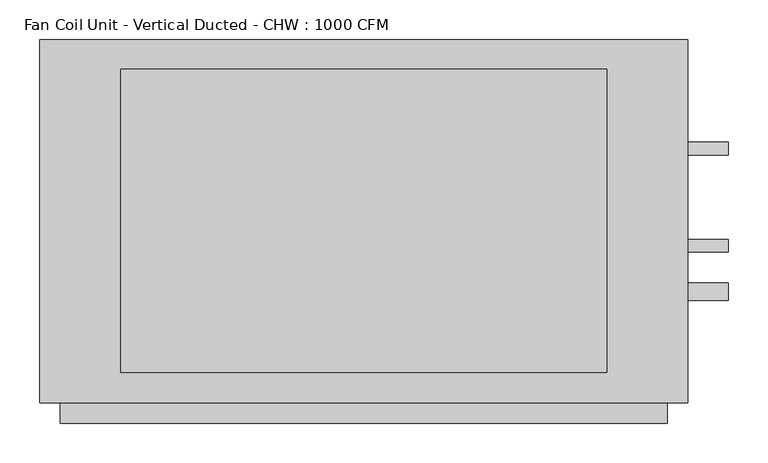
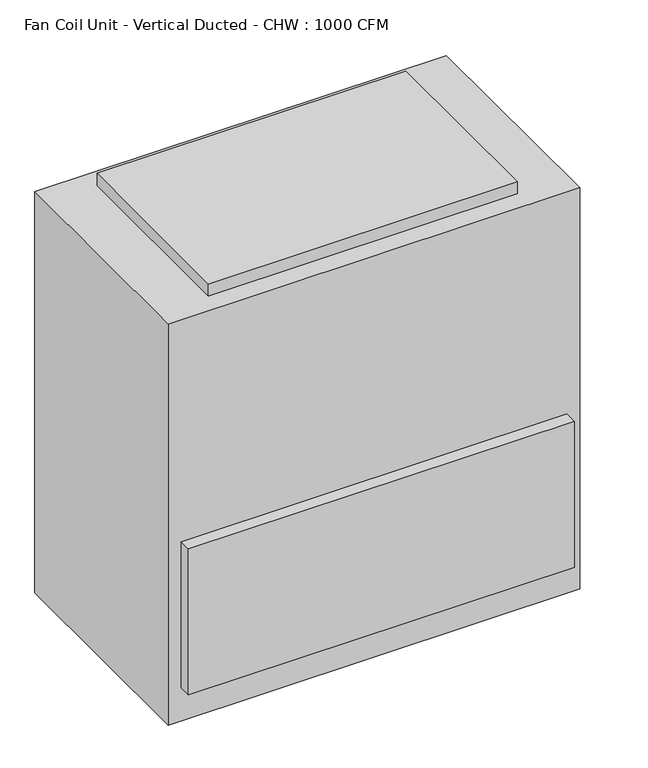
"""IFC4 building model written with IfcOpenShell, lengths in millimetres: proxy geometry, Fan Coil Unit - Vertical Ducted - CHW : 1000 CFM."""

from ifc_helpers import new_model, si_unit, frame, origin, place, context, project, spatial, circle_curve, source, transform, mapped, element, save
from ifc_brep_helpers import plane_surface, cylinder_surface, advanced_brep


def fan_coil_unit_vertical_ducted_chw_1000_cfm_3afe99c5(model_context):
    return source(origin(), model_context, "Body", "AdvancedBrep", [
        advanced_brep(
        [(711.2, 419.1, 863.6), (101.6, 419.1, 863.6), (101.6, 38.1, 863.6), (711.2, 38.1, 863.6), (711.2, 419.1, 838.2), (101.6, 419.1, 838.2), (101.6, 38.1, 838.2), (711.2, 38.1, 838.2), (812.8, 455.901774, 838.2), (0.0, 455.901774, 838.2), (0.0, 0.0, 838.2), (812.8, 0.0, 838.2), (812.8, 455.901774, 0.0), (812.8, 0.0, 0.0), (0.0, 0.0, 0.0), (0.0, 455.901774, 0.0), (25.4, 0.0, 374.65), (787.4, 0.0, 374.65), (787.4, 0.0, 69.85), (25.4, 0.0, 69.85), (812.8, 327.314274, 673.1), (812.8, 311.439274, 673.1), (812.8, 205.076774, 593.725), (812.8, 189.201774, 593.725), (812.8, 150.8125, 431.8), (812.8, 128.5875, 431.8), (787.4, -25.4, 374.65), (25.4, -25.4, 374.65), (25.4, -25.4, 69.85), (787.4, -25.4, 69.85), (863.6, 311.439274, 673.1), (863.6, 327.314274, 673.1), (863.6, 189.201774, 593.725), (863.6, 205.076774, 593.725), (863.6, 128.5875, 431.8), (863.6, 150.8125, 431.8)],
        [
            (0, 1),
            (1, 2),
            (2, 3),
            (3, 0),
            (0, 4),
            (4, 5),
            (5, 1),
            (5, 6),
            (6, 2),
            (6, 7),
            (7, 3),
            (7, 4),
            (8, 9),
            (9, 10),
            (10, 11),
            (11, 8),
            (12, 13),
            (13, 14),
            (14, 15),
            (15, 12),
            (8, 12),
            (15, 9),
            (14, 10),
            (13, 11),
            (16, 17),
            (17, 18),
            (18, 19),
            (19, 16),
            (20, 21, circle_curve(frame((812.8, 319.376774, 673.1), z_axis=(-1.0, 0.0, 0.0), x_axis=(0.0, 1.0, 0.0)), 7.9375)),
            (21, 20, circle_curve(frame((812.8, 319.376774, 673.1), z_axis=(-1.0, 0.0, 0.0), x_axis=(0.0, 1.0, 0.0)), 7.9375)),
            (22, 23, circle_curve(frame((812.8, 197.139274, 593.725), z_axis=(-1.0, 0.0, 0.0), x_axis=(0.0, 1.0, 0.0)), 7.9375)),
            (23, 22, circle_curve(frame((812.8, 197.139274, 593.725), z_axis=(-1.0, 0.0, 0.0), x_axis=(0.0, 1.0, 0.0)), 7.9375)),
            (24, 25, circle_curve(frame((812.8, 139.7, 431.8), z_axis=(-1.0, 0.0, 0.0), x_axis=(0.0, 1.0, 0.0)), 11.1125)),
            (25, 24, circle_curve(frame((812.8, 139.7, 431.8), z_axis=(-1.0, 0.0, 0.0), x_axis=(0.0, 1.0, 0.0)), 11.1125)),
            (26, 27),
            (27, 28),
            (28, 29),
            (29, 26),
            (26, 17),
            (16, 27),
            (19, 28),
            (18, 29),
            (30, 31, circle_curve(frame((863.6, 319.376774, 673.1), z_axis=(1.0, 0.0, 0.0), x_axis=(0.0, 1.0, 0.0)), 7.9375)),
            (31, 30, circle_curve(frame((863.6, 319.376774, 673.1), z_axis=(1.0, 0.0, 0.0), x_axis=(0.0, 1.0, 0.0)), 7.9375)),
            (30, 21),
            (20, 31),
            (32, 33, circle_curve(frame((863.6, 197.139274, 593.725), z_axis=(1.0, 0.0, 0.0), x_axis=(0.0, 1.0, 0.0)), 7.9375)),
            (33, 32, circle_curve(frame((863.6, 197.139274, 593.725), z_axis=(1.0, 0.0, 0.0), x_axis=(0.0, 1.0, 0.0)), 7.9375)),
            (32, 23),
            (22, 33),
            (34, 35, circle_curve(frame((863.6, 139.7, 431.8), z_axis=(1.0, 0.0, 0.0), x_axis=(0.0, 1.0, 0.0)), 11.1125)),
            (35, 34, circle_curve(frame((863.6, 139.7, 431.8), z_axis=(1.0, 0.0, 0.0), x_axis=(0.0, 1.0, 0.0)), 11.1125)),
            (34, 25),
            (24, 35),
        ],
        [
            plane_surface(frame((101.6, 419.1, 863.6), z_axis=(0.0, 0.0, 1.0), x_axis=(-1.0, 0.0, 0.0))),
            plane_surface(frame((711.2, 419.1, 863.6), z_axis=(0.0, 1.0, 0.0), x_axis=(0.0, 0.0, -1.0))),
            plane_surface(frame((101.6, 419.1, 863.6), z_axis=(-1.0, 0.0, 0.0), x_axis=(0.0, 0.0, -1.0))),
            plane_surface(frame((101.6, 38.1, 863.6), z_axis=(0.0, -1.0, 0.0), x_axis=(0.0, 0.0, -1.0))),
            plane_surface(frame((711.2, 38.1, 863.6), z_axis=(1.0, 0.0, 0.0), x_axis=(0.0, 0.0, -1.0))),
            plane_surface(frame((0.0, 455.901774, 838.2), z_axis=(0.0, 0.0, 1.0), x_axis=(-1.0, 0.0, 0.0))),
            plane_surface(frame((0.0, 455.901774, 0.0), z_axis=(0.0, 0.0, -1.0), x_axis=(1.0, 0.0, 0.0))),
            plane_surface(frame((812.8, 455.901774, 838.2), z_axis=(0.0, 1.0, 0.0), x_axis=(0.0, 0.0, -1.0))),
            plane_surface(frame((0.0, 455.901774, 838.2), z_axis=(-1.0, 0.0, 0.0), x_axis=(0.0, 0.0, -1.0))),
            plane_surface(frame((0.0, 0.0, 838.2), z_axis=(0.0, -1.0, 0.0), x_axis=(0.0, 0.0, -1.0))),
            plane_surface(frame((812.8, 0.0, 838.2), z_axis=(1.0, 0.0, 0.0), x_axis=(0.0, 0.0, -1.0))),
            plane_surface(frame((25.4, -25.4, 374.65), z_axis=(0.0, -1.0, 0.0), x_axis=(-1.0, 0.0, 0.0))),
            plane_surface(frame((787.4, -25.4, 374.65), z_axis=(0.0, 0.0, 1.0), x_axis=(0.0, 1.0, 0.0))),
            plane_surface(frame((25.4, -25.4, 374.65), z_axis=(-1.0, 0.0, 0.0), x_axis=(0.0, 1.0, 0.0))),
            plane_surface(frame((25.4, -25.4, 69.85), z_axis=(0.0, 0.0, -1.0), x_axis=(0.0, 1.0, 0.0))),
            plane_surface(frame((787.4, -25.4, 69.85), z_axis=(1.0, 0.0, 0.0), x_axis=(0.0, 1.0, 0.0))),
            plane_surface(frame((863.6, 327.314274, 673.1), z_axis=(1.0, 0.0, 0.0), x_axis=(0.0, 0.0, 1.0))),
            cylinder_surface(frame((812.8, 319.376774, 673.1), z_axis=(1.0, 0.0, 0.0), x_axis=(0.0, 1.0, 0.0)), 7.9375),
            plane_surface(frame((863.6, 205.076774, 593.725), z_axis=(1.0, 0.0, 0.0), x_axis=(0.0, 0.0, 1.0))),
            cylinder_surface(frame((812.8, 197.139274, 593.725), z_axis=(1.0, 0.0, 0.0), x_axis=(0.0, 1.0, 0.0)), 7.9375),
            plane_surface(frame((863.6, 150.8125, 431.8), z_axis=(1.0, 0.0, 0.0), x_axis=(0.0, 0.0, 1.0))),
            cylinder_surface(frame((812.8, 139.7, 431.8), z_axis=(1.0, 0.0, 0.0), x_axis=(0.0, 1.0, 0.0)), 11.1125),
        ],
        [
            (0, [[1, 2, 3, 4]]),
            (1, [[-1, 5, 6, 7]]),
            (2, [[-2, -7, 8, 9]]),
            (3, [[-3, -9, 10, 11]]),
            (4, [[-4, -11, 12, -5]]),
            (5, [[13, 14, 15, 16], [-6, -12, -10, -8]]),
            (6, [[17, 18, 19, 20]]),
            (7, [[-13, 21, -20, 22]]),
            (8, [[-14, -22, -19, 23]]),
            (9, [[-15, -23, -18, 24], [25, 26, 27, 28]]),
            (10, [[-16, -24, -17, -21], [29, 30], [31, 32], [33, 34]]),
            (11, [[35, 36, 37, 38]]),
            (12, [[-35, 39, -25, 40]]),
            (13, [[-36, -40, -28, 41]]),
            (14, [[-37, -41, -27, 42]]),
            (15, [[-38, -42, -26, -39]]),
            (16, [[43, 44]]),
            (17, [[-43, 45, -29, 46]]),
            (17, [[-44, -46, -30, -45]]),
            (18, [[47, 48]]),
            (19, [[-47, 49, -31, 50]]),
            (19, [[-48, -50, -32, -49]]),
            (20, [[51, 52]]),
            (21, [[-51, 53, -33, 54]]),
            (21, [[-52, -54, -34, -53]]),
        ],
    ),
    ])


if __name__ == "__main__":
    model = new_model("IFC4")
    model_context = context("Model", 3, world=origin())
    ifc_project = project(units=[si_unit("LENGTHUNIT", "METRE", prefix="MILLI")], contexts=[model_context])
    site = spatial("IfcSite", under=ifc_project)
    building = spatial("IfcBuilding", under=site)
    placement = place(None, origin())
    fan_coil_unit_vertical_ducted_chw_1000_cfm_shape = fan_coil_unit_vertical_ducted_chw_1000_cfm_3afe99c5(model_context)
    element("IfcBuildingElementProxy", 1, Name="Fan Coil Unit - Vertical Ducted - CHW : 1000 CFM", ObjectType="Fan Coil Unit - Vertical Ducted - CHW : 1000 CFM", at=placement, inside=building, context=model_context, shape_type="MappedRepresentation", body=[
        mapped(fan_coil_unit_vertical_ducted_chw_1000_cfm_shape, transform((0.0, 0.0, 0.0), x_axis=(1.0, 0.0, 0.0), y_axis=(0.0, 1.0, 0.0), z_axis=(0.0, 0.0, 1.0))),
    ])
    save(model, "model.ifc")

# Revit data of these elements
# Type "Fan Coil Unit - Vertical Ducted - CHW : 1000 CFM"
#   COBie.Type.CreatedBy = "design@eagle.com"
#   COBie.Type.CreatedOn = "2016-10-27T05:31:12"
#   COBie.Type.Name = "Fan Coil Unit - Vertical Ducted - CHW_1000 CFM"
#   COBie.Type.Category = "23-75 70 17 27 : Fan Coil Units"
#   COBie.Type.Description = "Fan Coil Unit - Vertical Ducted - CHW_1000 CFM"
#   COBie.Type.Manufacturer = ""
#   COBie.Type.ModelNumber = ""
#   COBie.Type.ReplacementCost = 0
#   Water Pressure Drop [instance default] = 6.50 psi
#   Voltage = 240 V
#   Unit Length = 2' - 8"
#   Total Cooling Capacity = 38500 Btu/h
#   Supply Air Width = 24"
#   Sensible Cooling Capacity = 26400 Btu/h
#   Return Air Width = 30"
#   Nominal Air Flow [instance default] = 1000 CFM
#   External Static Pressure [instance default] = 0.30 in-wg
#   Drain Flow [instance default] = 0 GPM
#   Chilled Water Flow [instance default] = 8 GPM
#   C2 Offset 1 = 0' - 5 3/8"
#   Apparent Load = 440 VA
#   COBie.Type = yes
#   Number of Poles = 2
#   Load Classification = Cooling
#   CFU Material = none
